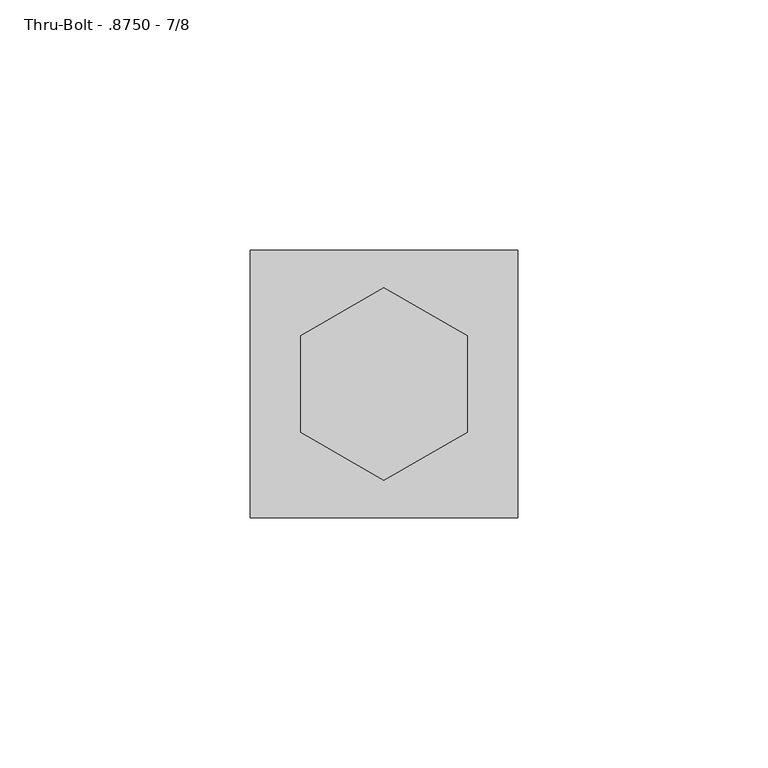
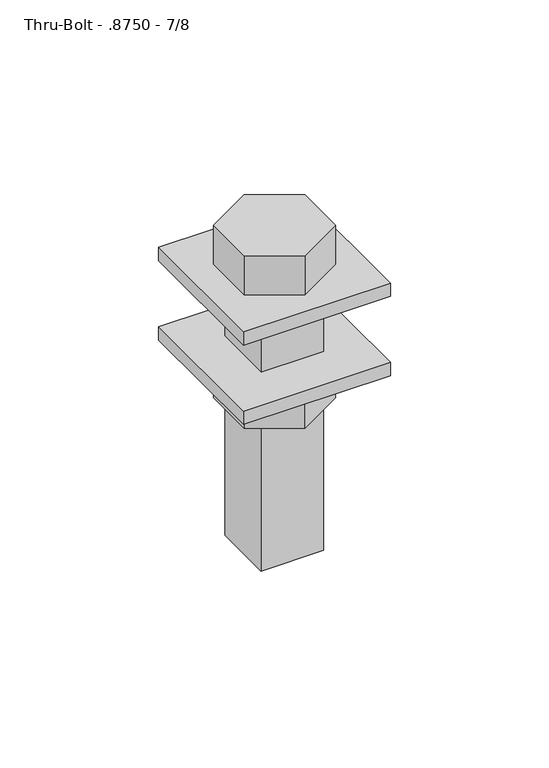
"""IFC4 building model written with IfcOpenShell, lengths in millimetres: fastener geometry, 060523 - W_P_C - Fastenings - Generic - SQUARE : Thru-Bolt - .8750 - 7/8."""

from ifc_helpers import new_model, si_unit, frame, origin, origin_with_axes, place, context, project, spatial, polyline, outline, extrude, source, transform, mapped, element, save


def thru_bolt_8750_7_8_31252657(model_context):
    return source(origin(), model_context, "Body", "SweptSolid", [
        extrude(outline(polyline([(-26.7394531, -26.7394531), (-26.7394531, 26.7394531), (26.7394531, 26.7394531), (26.7394531, -26.7394531), (-26.7394531, -26.7394531)])), origin_with_axes(), (0.0, 0.0, 1.0), 5.1263021),
        extrude(outline(polyline([(-26.7394531, -26.7394531), (-26.7394531, 26.7394531), (26.7394531, 26.7394531), (26.7394531, -26.7394531), (-26.7394531, -26.7394531)])), frame((0.0, 0.0, -30.5263021), z_axis=(0.0, 0.0, 1.0), x_axis=(1.0, 0.0, 0.0)), (0.0, 0.0, 1.0), 5.1263021),
        extrude(outline(polyline([(-16.66875, -9.6237073), (-16.66875, 9.6237073), (0.0, 19.2474146), (16.66875, 9.6237073), (16.66875, -9.6237073), (0.0, -19.2474146), (-16.66875, -9.6237073)])), frame((0.0, 0.0, -45.9052083), z_axis=(0.0, 0.0, 1.0), x_axis=(1.0, 0.0, 0.0)), (0.0, 0.0, 1.0), 15.3789062),
        extrude(outline(polyline([(-16.66875, 9.6237073), (0.0, 19.2474146), (16.66875, 9.6237073), (16.66875, -9.6237073), (0.0, -19.2474146), (-16.66875, -9.6237073), (-16.66875, 9.6237073)])), frame((0.0, 0.0, 5.1263021), z_axis=(0.0, 0.0, 1.0), x_axis=(1.0, 0.0, 0.0)), (0.0, 0.0, 1.0), 15.3789062),
        extrude(outline(polyline([(-11.3605469, 11.3605469), (11.3605469, 11.3605469), (11.3605469, -11.3605469), (-11.3605469, -11.3605469), (-11.3605469, 11.3605469)])), frame((0.0, 0.0, -101.6), z_axis=(0.0, 0.0, 1.0), x_axis=(1.0, 0.0, 0.0)), (0.0, 0.0, 1.0), 106.7263021),
    ])


if __name__ == "__main__":
    model = new_model("IFC4")
    model_context = context("Model", 3, world=origin())
    ifc_project = project(units=[si_unit("LENGTHUNIT", "METRE", prefix="MILLI")], contexts=[model_context])
    site = spatial("IfcSite", under=ifc_project)
    building = spatial("IfcBuilding", under=site)
    placement = place(None, origin())
    thru_bolt_8750_7_8_shape = thru_bolt_8750_7_8_31252657(model_context)
    element("IfcFastener", 1, ObjectType="060523 - W_P_C - Fastenings - Generic - SQUARE : Thru-Bolt - .8750 - 7/8", at=placement, inside=building, context=model_context, shape_type="MappedRepresentation", body=[
        mapped(thru_bolt_8750_7_8_shape, transform((0.0, 0.0, 0.0), x_axis=(1.0, 0.0, 0.0), y_axis=(0.0, 1.0, 0.0), z_axis=(0.0, 0.0, 1.0))),
    ])
    save(model, "model.ifc")

# Revit data of these elements
# Type "060523 - W_P_C - Fastenings - Generic - SQUARE : Thru-Bolt - .8750 - 7/8"
#   Washer_Thickness = 0' - 0.20182"
#   Washer Radius = 0' - 1.05273"
#   Washer Offset - Head = 0' - 0.20182"
#   Washer Offset = 0' - 0.20182"
#   Thickness_of_Substrate [instance default] = 0' - 1"
#   Side = 0' - 0.75879"
#   Radius = 0' - 0.44727"
#   Length [instance default] = 0' - 4"
#   Head Size = 0' - 1 5/16"
#   Head Radius = 0' - 0 21/32"
#   Head Height = 0' - 0 155/256"
#   Double Diameter = 0' - 1 101/128"
#   Diameter = 0' - 0 229/256"
#   Default Elevation = 4' - 0"
#   Washer_Nut_Visibility = yes
#   Washer_Head_Visibility = yes
#   Round_Head_Visibility = no
#   Point Visibility = no
#   Nut_Visibility = yes
#   Hex_Head_Visiblilty = yes
#   Washer Material = none
#   Bolt Material (Size) = AT SILL - FASTENER AT 24" O.C.
# Element 1 (IfcFastener, "060523 - W_P_C - Fastenings - Generic - SQUARE : Thru-Bolt - .8750 - 7/8")
#   Materials on its faces: "AT SILL - FASTENER AT 24\" O.C."
# Materials
#   "AT SILL - FASTENER AT 24\" O.C.": class "Generic", colour RGB 120 120 120, transparency 0, Cost = 0
